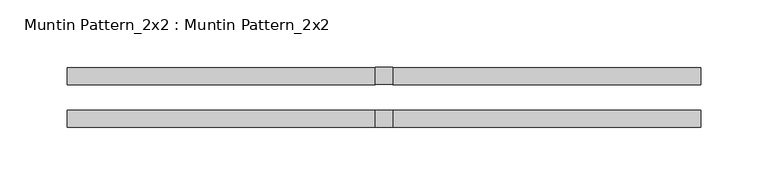
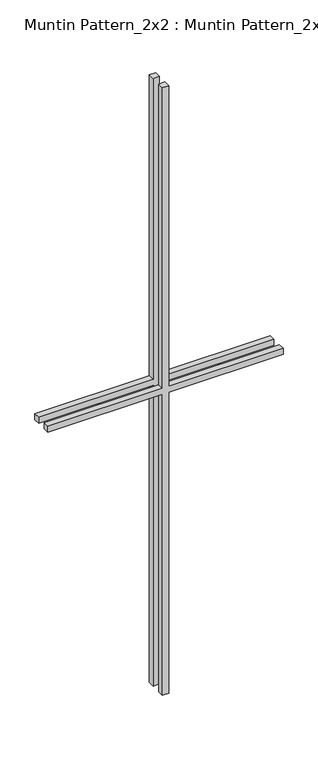
"""IFC4 building model written with IfcOpenShell, lengths in millimetres: proxy geometry, Muntin Pattern_2x2 : Muntin Pattern_2x2."""

from ifc_helpers import new_model, si_unit, frame, origin, place, context, project, spatial, polyline, outline, extrude, source, transform, mapped, element, save


def muntin_pattern_2x2_muntin_pattern_2x2_5bc79d00(model_context):
    return source(origin(), model_context, "Body", "SweptSolid", [
        extrude(outline(polyline([(647.7, -6.35), (647.7, -234.95), (635.0, -234.95), (635.0, -6.35), (0.0, -6.35), (0.0, 6.35), (635.0, 6.35), (635.0, 234.95), (647.7, 234.95), (647.7, 6.35), (1282.7, 6.35), (1282.7, -6.35), (647.7, -6.35)])), frame((0.0, -22.225, 0.0), z_axis=(0.0, 1.0, 0.0), x_axis=(0.0, 0.0, 1.0)), (0.0, 0.0, 1.0), 12.7),
        extrude(outline(polyline([(647.7, -6.35), (647.7, -234.95), (635.0, -234.95), (635.0, -6.35), (0.0, -6.35), (0.0, 6.35), (635.0, 6.35), (635.0, 234.95), (647.7, 234.95), (647.7, 6.35), (1282.7, 6.35), (1282.7, -6.35), (647.7, -6.35)])), frame((0.0, 9.525, 0.0), z_axis=(0.0, 1.0, 0.0), x_axis=(0.0, 0.0, 1.0)), (0.0, 0.0, 1.0), 12.7),
    ])


if __name__ == "__main__":
    model = new_model("IFC4")
    model_context = context("Model", 3, world=origin())
    ifc_project = project(units=[si_unit("LENGTHUNIT", "METRE", prefix="MILLI")], contexts=[model_context])
    site = spatial("IfcSite", under=ifc_project)
    building = spatial("IfcBuilding", under=site)
    placement = place(None, origin())
    muntin_pattern_2x2_muntin_pattern_2x2_shape = muntin_pattern_2x2_muntin_pattern_2x2_5bc79d00(model_context)
    element("IfcBuildingElementProxy", 1, Name="Muntin Pattern_2x2 : Muntin Pattern_2x2", ObjectType="Muntin Pattern_2x2 : Muntin Pattern_2x2", at=placement, inside=building, context=model_context, shape_type="MappedRepresentation", body=[
        mapped(muntin_pattern_2x2_muntin_pattern_2x2_shape, transform((0.0, 0.0, 0.0), x_axis=(1.0, 0.0, 0.0), y_axis=(0.0, 1.0, 0.0), z_axis=(0.0, 0.0, 1.0))),
    ])
    save(model, "model.ifc")

# Revit data of these elements
# Type "Muntin Pattern_2x2 : Muntin Pattern_2x2"
#   Width [instance default] = 4' - 0"
#   Thickness = 0' - 0 1/2"
#   Height [instance default] = 4' - 0"
#   Distance = 0' - 0 3/4"
#   Interior Material [instance default] = none
#   Exterior Material [instance default] = none
#   Default Elevation = 0
# Element 1 (IfcBuildingElementProxy, "Muntin Pattern_2x2 : Muntin Pattern_2x2")
#   Width = 1' - 6 1/2"
#   Height = 4' - 2 1/2"
#   Interior Material = Maple - Semigloss(Rotated)
#   Exterior Material = Clad - White
#   Materials on its faces: "Clad - White", "Maple - Semigloss(Rotated)"
# Materials
#   "Clad - White": class "Wood", colour RGB 245 245 243, transparency 0, Cost = 0
#   "Maple - Semigloss(Rotated)": class "Wood", colour RGB 196 161 118, transparency 0, Description = "Acer Saccharum", Cost = 0
